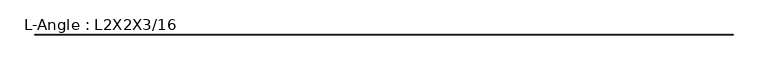
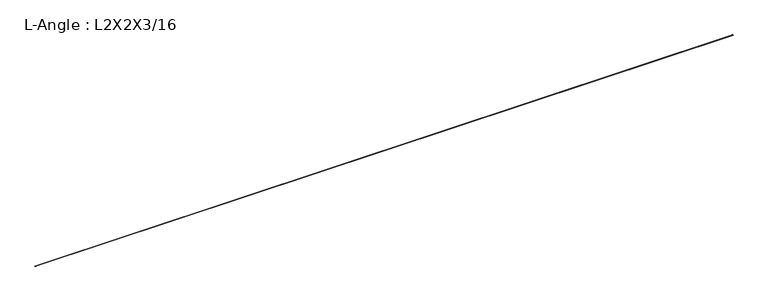
"""IFC4 building model written with IfcOpenShell, lengths in millimetres: beam geometry, L-Angle : L2X2X3/16."""

from ifc_helpers import new_model, si_unit, point, frame, frame_2d, origin, place, context, project, spatial, polyline, circle_curve, trimmed, segment, composite_curve, outline, extrude, source, transform, mapped, element, save


def l_angle_l2x2x3_16_cd50c46b(model_context):
    return source(origin(), model_context, "Body", "SweptSolid", [
        extrude(outline(composite_curve([segment(polyline([(14.2494, 14.2494), (14.2494, -36.5506)]), True, "CONTINUOUS"), segment(trimmed(circle_curve(frame_2d((14.2494, -31.7881)), 4.7625), [point((14.2494, -36.5506))], [point((9.4869, -31.7881))], False, "CARTESIAN"), True, "CONTINUOUS"), segment(polyline([(9.4869, -31.7881), (9.4869, 4.7244)]), True, "CONTINUOUS"), segment(trimmed(circle_curve(frame_2d((4.7244, 4.7244)), 4.7625), [point((9.4869, 4.7244))], [point((4.7244, 9.4869))], True, "CARTESIAN"), True, "CONTINUOUS"), segment(polyline([(4.7244, 9.4869), (-31.7881, 9.4869)]), True, "CONTINUOUS"), segment(trimmed(circle_curve(frame_2d((-31.7881, 14.2494)), 4.7625), [point((-31.7881, 9.4869))], [point((-36.5506, 14.2494))], False, "CARTESIAN"), True, "CONTINUOUS"), segment(polyline([(-36.5506, 14.2494), (14.2494, 14.2494)]), True, "CONTINUOUS")], self_intersect=False)), frame((-44323.0, 0.0, 0.0), z_axis=(1.0, 0.0, 0.0), x_axis=(0.0, 1.0, 0.0)), (0.0, 0.0, 1.0), 88430.1),
    ])


if __name__ == "__main__":
    model = new_model("IFC4")
    model_context = context("Model", 3, world=origin())
    ifc_project = project(units=[si_unit("LENGTHUNIT", "METRE", prefix="MILLI")], contexts=[model_context])
    site = spatial("IfcSite", under=ifc_project)
    building = spatial("IfcBuilding", under=site)
    placement = place(None, origin())
    l_angle_l2x2x3_16_shape = l_angle_l2x2x3_16_cd50c46b(model_context)
    element("IfcBeam", 1, ObjectType="L-Angle : L2X2X3/16", at=placement, inside=building, context=model_context, shape_type="MappedRepresentation", body=[
        mapped(l_angle_l2x2x3_16_shape, transform((0.0, 0.0, 0.0), x_axis=(1.0, 0.0, 0.0), y_axis=(0.0, 1.0, 0.0), z_axis=(0.0, 0.0, 1.0))),
    ])
    save(model, "model.ifc")

# Revit data of these elements
# Type "L-Angle : L2X2X3/16"
#   Assembly Code = "B10"
#   k = 0' - 0 7/16"
#   W = 2.44
#   Start Extension Calculation [instance default] = 10' - 0"
#   Start Extension [instance default] = -0' - 0 1/2"
#   End Extension Calculation [instance default] = 10' - 0"
#   End Extension [instance default] = -0' - 0 1/2"
#   Length [instance default] = 5' - 0"
#   b = 0' - 2"
#   d = 0' - 2"
#   t = 0' - 0 3/16"
#   x = 0' - 0.561"
#   y = 0' - 0.561"
#   A = 0.00496528 SF
#   Structural Material [instance default] = Metal - Steel - ASTM A36
# Element 1 (IfcBeam, "L-Angle : L2X2X3/16")
#   Structural Material = STRUCTURAL STEEL - SEE STRUCT. DWGS
#   Materials on its faces: "STRUCTURAL STEEL - SEE STRUCT. DWGS"
# Materials
#   "Metal - Steel - ASTM A36": class "Metal", colour RGB 199 199 199, transparency 0
#   "STRUCTURAL STEEL - SEE STRUCT. DWGS": class "Metal", colour RGB 137 146 153, transparency 0, Description = "Steel, mill finish", Cost = 0
